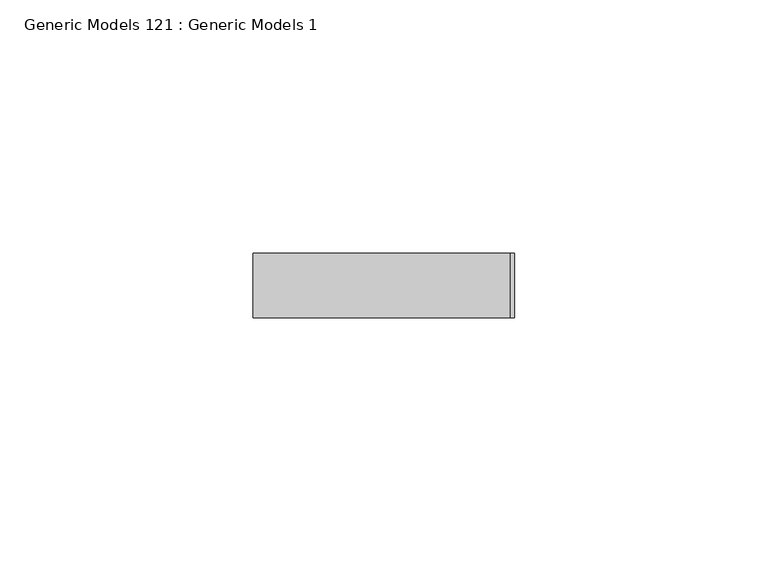
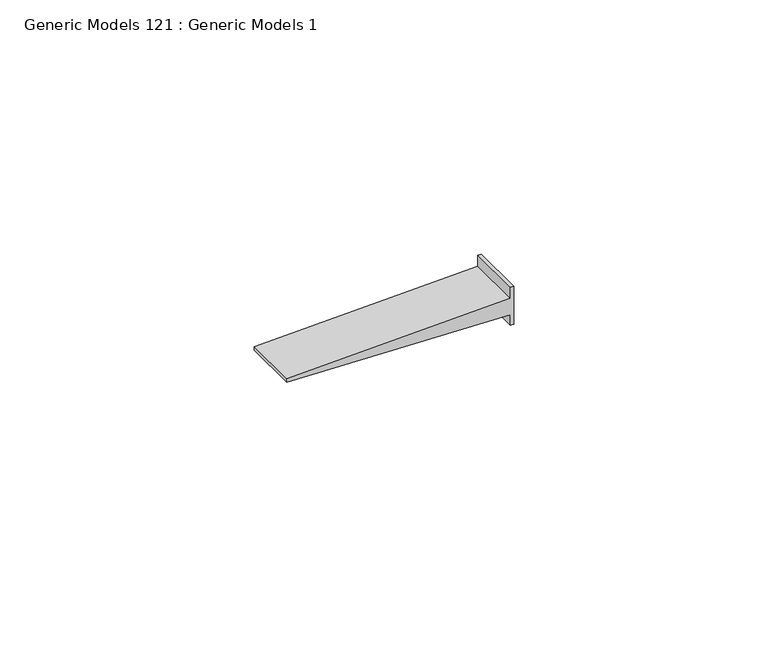
"""IFC4 building model written with IfcOpenShell, lengths in millimetres: proxy geometry, Generic Models 121 : Generic Models 1."""

from ifc_helpers import new_model, si_unit, frame, origin, place, context, project, spatial, polyline, outline, extrude, source, transform, mapped, element, save


def generic_models_121_generic_models_1_6df95633(model_context):
    return source(origin(), model_context, "Body", "SweptSolid", [
        extrude(outline(polyline([(259.1857124, 49818.9869139), (259.1857124, 49818.1931639), (256.6358488, 49818.1931639), (255.0384597, 49767.3931639), (254.2397651, 49767.3931639), (252.642376, 49818.1931639), (250.0925124, 49818.1931639), (250.0925124, 49818.9869139), (259.1857124, 49818.9869139)])), frame((0.0, 565.15, 0.0), z_axis=(0.0, 1.0, 0.0), x_axis=(0.0, 0.0, 1.0)), (0.0, 0.0, 1.0), 12.7),
    ])


if __name__ == "__main__":
    model = new_model("IFC4")
    model_context = context("Model", 3, world=origin())
    ifc_project = project(units=[si_unit("LENGTHUNIT", "METRE", prefix="MILLI")], contexts=[model_context])
    site = spatial("IfcSite", under=ifc_project)
    building = spatial("IfcBuilding", under=site)
    placement = place(None, origin())
    generic_models_121_generic_models_1_shape = generic_models_121_generic_models_1_6df95633(model_context)
    element("IfcBuildingElementProxy", 1, Name="Generic Models 121 : Generic Models 1", ObjectType="Generic Models 121 : Generic Models 1", at=placement, inside=building, context=model_context, shape_type="MappedRepresentation", body=[
        mapped(generic_models_121_generic_models_1_shape, transform((0.0, 0.0, 0.0), x_axis=(1.0, 0.0, 0.0), y_axis=(0.0, 1.0, 0.0), z_axis=(0.0, 0.0, 1.0))),
    ])
    save(model, "model.ifc")

# Revit data of these elements
# Element 1 (IfcBuildingElementProxy, "Generic Models 121 : Generic Models 1")
#   Materials on its faces: "ATTACH GYPSUM BOARD TO STUDS AND NOT TO TOP TRACK"
# Materials
#   "ATTACH GYPSUM BOARD TO STUDS AND NOT TO TOP TRACK": class "Generic", colour RGB 48 48 48, transparency 0, Cost = 0
